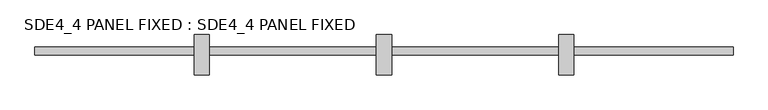
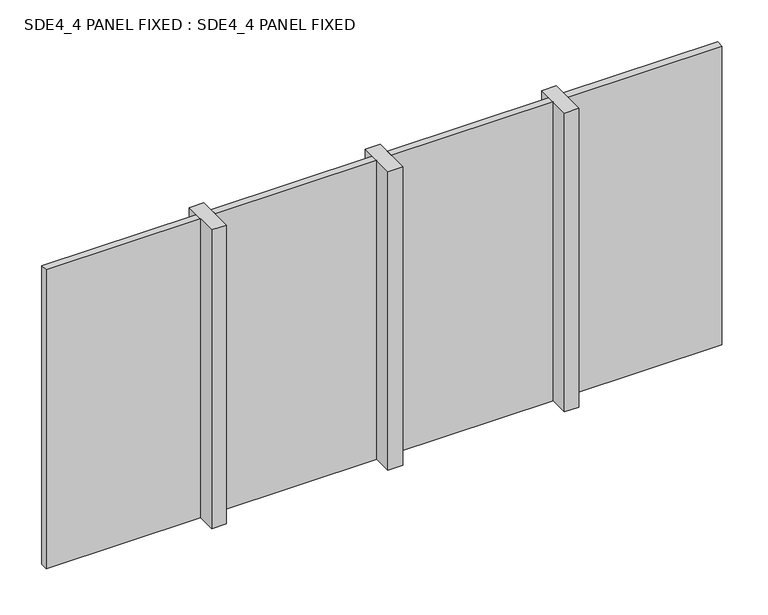
"""IFC4 building model written with IfcOpenShell, lengths in millimetres: plate geometry, SDE4_4 PANEL FIXED : SDE4_4 PANEL FIXED."""

from ifc_helpers import new_model, si_unit, origin, origin_with_axes, place, context, project, spatial, polyline, outline, extrude, source, transform, mapped, element, save


def sde4_4_panel_fixed_sde4_4_panel_fixed_9ab70056(model_context):
    return source(origin(), model_context, "Body", "SweptSolid", [
        extrude(outline(polyline([(-1150.0, 132.5), (-1150.0, -132.5), (-1250.0, -132.5), (-1250.0, 132.5), (-1150.0, 132.5)])), origin_with_axes(), (0.0, 0.0, 1.0), 2150.0),
        extrude(outline(polyline([(50.0, 132.5), (50.0, -132.5), (-50.0, -132.5), (-50.0, 132.5), (50.0, 132.5)])), origin_with_axes(), (0.0, 0.0, 1.0), 2150.0),
        extrude(outline(polyline([(1250.0, 132.5), (1250.0, -132.5), (1150.0, -132.5), (1150.0, 132.5), (1250.0, 132.5)])), origin_with_axes(), (0.0, 0.0, 1.0), 2150.0),
        extrude(outline(polyline([(2299.0, 50.0), (2299.0, 0.0), (1250.0, 0.0), (1250.0, 50.0), (2299.0, 50.0)])), origin_with_axes(), (0.0, 0.0, 1.0), 2150.0),
        extrude(outline(polyline([(1150.0, 50.0), (1150.0, 0.0), (50.0, 0.0), (50.0, 50.0), (1150.0, 50.0)])), origin_with_axes(), (0.0, 0.0, 1.0), 2150.0),
        extrude(outline(polyline([(-50.0, 50.0), (-50.0, 0.0), (-1150.0, 0.0), (-1150.0, 50.0), (-50.0, 50.0)])), origin_with_axes(), (0.0, 0.0, 1.0), 2150.0),
        extrude(outline(polyline([(-1250.0, 50.0), (-1250.0, 0.0), (-2300.0, 0.0), (-2300.0, 50.0), (-1250.0, 50.0)])), origin_with_axes(), (0.0, 0.0, 1.0), 2150.0),
    ])


if __name__ == "__main__":
    model = new_model("IFC4")
    model_context = context("Model", 3, world=origin())
    ifc_project = project(units=[si_unit("LENGTHUNIT", "METRE", prefix="MILLI")], contexts=[model_context])
    site = spatial("IfcSite", under=ifc_project)
    building = spatial("IfcBuilding", under=site)
    placement = place(None, origin())
    sde4_4_panel_fixed_sde4_4_panel_fixed_shape = sde4_4_panel_fixed_sde4_4_panel_fixed_9ab70056(model_context)
    element("IfcPlate", 1, ObjectType="SDE4_4 PANEL FIXED : SDE4_4 PANEL FIXED", at=placement, inside=building, context=model_context, shape_type="MappedRepresentation", body=[
        mapped(sde4_4_panel_fixed_sde4_4_panel_fixed_shape, transform((0.0, 0.0, 0.0), x_axis=(1.0, 0.0, 0.0), y_axis=(0.0, 1.0, 0.0), z_axis=(0.0, 0.0, 1.0))),
    ])
    save(model, "model.ifc")

# Revit data of these elements
# Type "SDE4_4 PANEL FIXED : SDE4_4 PANEL FIXED"
#   Type Mark = "CW-GLASS"
#   Analytic Construction = "<None>"
#   Glass = Glass
#   Frame = Aluminium
# Element 1 (IfcPlate, "SDE4_4 PANEL FIXED : SDE4_4 PANEL FIXED")
#   Materials on its faces: "Glass", "Aluminium"
# Materials
#   "Glass": class "Glass", colour RGB 0 128 192, transparency 0.9, Keynote = "L40", Cost = 0
#   "Aluminium": class "Unassigned", colour RGB 247 247 247, transparency 0, Cost = 0
